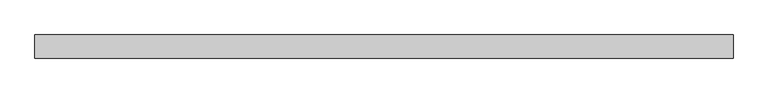
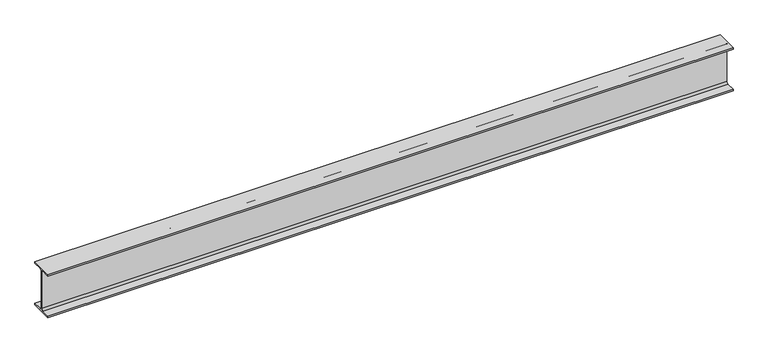
"""IFC4 building model written with IfcOpenShell, lengths in millimetres: beam geometry, 0912_Steel Framing_H-KSD3502 : H_SB_ASB_H-400x200x8x13."""

from ifc_helpers import new_model, si_unit, point, frame, frame_2d, origin, place, context, project, spatial, polyline, circle_curve, trimmed, segment, composite_curve, outline, extrude, source, transform, mapped, element, save


def beam_f8e41749(model_context):
    return source(origin(), model_context, "Body", "SweptSolid", [
        extrude(outline(composite_curve([segment(polyline([(100.0, -187.0), (100.0, -200.0), (-100.0, -200.0), (-100.0, -187.0), (-20.0, -187.0)]), True, "CONTINUOUS"), segment(trimmed(circle_curve(frame_2d((-20.0, -171.0)), 16.0), [point((-20.0, -187.0))], [point((-4.0, -171.0))], True, "CARTESIAN"), True, "CONTINUOUS"), segment(polyline([(-4.0, -171.0), (-4.0, 171.0)]), True, "CONTINUOUS"), segment(trimmed(circle_curve(frame_2d((-20.0, 171.0)), 16.0), [point((-4.0, 171.0))], [point((-20.0, 187.0))], True, "CARTESIAN"), True, "CONTINUOUS"), segment(polyline([(-20.0, 187.0), (-100.0, 187.0), (-100.0, 200.0), (100.0, 200.0), (100.0, 187.0), (20.0, 187.0)]), True, "CONTINUOUS"), segment(trimmed(circle_curve(frame_2d((20.0, 171.0)), 16.0), [point((20.0, 187.0))], [point((4.0, 171.0))], True, "CARTESIAN"), True, "CONTINUOUS"), segment(polyline([(4.0, 171.0), (4.0, -171.0)]), True, "CONTINUOUS"), segment(trimmed(circle_curve(frame_2d((20.0, -171.0)), 16.0), [point((4.0, -171.0))], [point((20.0, -187.0))], True, "CARTESIAN"), True, "CONTINUOUS"), segment(polyline([(20.0, -187.0), (100.0, -187.0)]), True, "CONTINUOUS")], self_intersect=False)), frame((-3007.3488581, 0.0, 0.0), z_axis=(1.0, 0.0, 0.0), x_axis=(0.0, 1.0, 0.0)), (0.0, 0.0, 1.0), 6044.6488581),
    ])


if __name__ == "__main__":
    model = new_model("IFC4")
    model_context = context("Model", 3, world=origin())
    ifc_project = project(units=[si_unit("LENGTHUNIT", "METRE", prefix="MILLI")], contexts=[model_context])
    site = spatial("IfcSite", under=ifc_project)
    building = spatial("IfcBuilding", under=site)
    placement = place(None, origin())
    beam_shape = beam_f8e41749(model_context)
    element("IfcBeam", 1, ObjectType="0912_Steel Framing_H-KSD3502 : H_SB_ASB_H-400x200x8x13", at=placement, inside=building, context=model_context, shape_type="MappedRepresentation", body=[
        mapped(beam_shape, transform((0.0, 0.0, 0.0), x_axis=(1.0, 0.0, 0.0), y_axis=(0.0, 1.0, 0.0), z_axis=(0.0, 0.0, 1.0))),
    ])
    save(model, "model.ifc")

# Revit data of these elements
# Type "0912_Steel Framing_H-KSD3502 : H_SB_ASB_H-400x200x8x13"
#   H_WM Code_1 = "S01AA002-00001 | Main Steel Structure Fabrication Work | Shelter/Building | Medium Steel - Standard (90KG/M>Weight≥30KG/M) | Material: (   )"
#   H_WM Code_2 = "S03AA028-00001 | Main Steel Structure Erection Work | Shelter/Building | Medium Steel (90KG/M>Weight≥30KG/M) | Material: (   )"
#   H_WM Code_3 = "S01AA010-00001 | Main Steel Structure Fabrication Work | Shelter/Building | Steel Painting/Coating | for Non-Fireproofed Steel Surface, Surface Preparation, Primer, Second & Final Coat | Material: (   )"
#   H_Q'ty Cal Type Tag = "SB-Q2"
#   Width = 20.0 cm
#   Web Thickness = 0.8 cm
#   Web Fillet = 1.6 cm
#   Warping Constant = 649000.0 cm⁶
#   W = 0
#   Torsional Moment of Inertia = 35.8981 cm⁴
#   Section Area = 84.12 cm²
#   Plastic Modulus weak axis = 268.0 cm³
#   Plastic Modulus strong axis = 1330.0 cm³
#   Perimeter = 1.56 m²/m
#   Nominal Weight = 66.00 kgf/m
#   Moment of Inertia weak axis = 1740.00 cm⁴
#   Moment of Inertia strong axis = 23700.00 cm⁴
#   Height = 40.0 cm
#   Flange Thickness = 1.3 cm
#   Elastic Modulus weak axis = 174.0 cm³
#   Elastic Modulus strong axis = 1190.0 cm³
#   Centroid Vertical = 20.0 cm
#   Centroid Horizontal = 10.0 cm
#   Ix = 237000000
#   Length [instance default] = 1.5240 m
#   Zx = 1330000
#   b = 0.2000 m
#   h = 0.4000 m
#   r = 0.0160 m
#   s = 0.0080 m
#   t = 0.0130 m
#   A = 0.008412 m²
#   Structural Material [instance default] = Steel, 45-345
#   Assembly Code = ""
# Element 1 (IfcBeam, "0912_Steel Framing_H-KSD3502 : H_SB_ASB_H-400x200x8x13")
#   Structural Material = none
# Materials
#   "Steel, 45-345": class "Metal", colour RGB 189 187 185, transparency 0, Description = "Steel 345 MPa", Cost = 0
